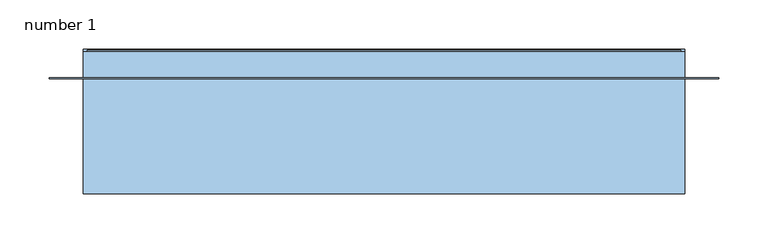
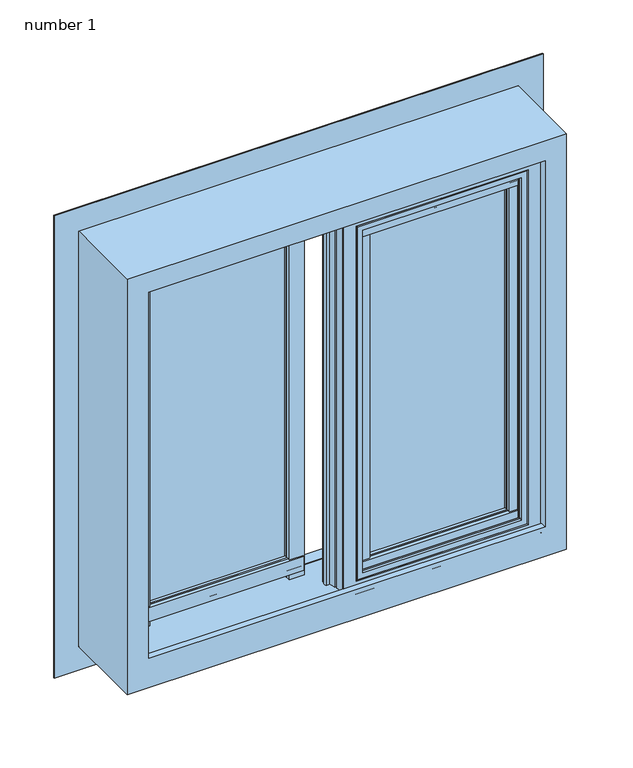
"""IFC4 building model written with IfcOpenShell, lengths in millimetres: window geometry, Window-Exterior-Sierra-Horizontal_Sliding_XO-36inch_Width-Standard : number 1."""

from ifc_helpers import new_model, si_unit, point, frame, frame_2d, origin, place, context, project, spatial, polyline, circle_curve, ellipse_curve, trimmed, segment, composite_curve, outline, extrude, faceted_brep, source, transform, mapped, element, save
from ifc_brep_helpers import plane_surface, cylinder_surface, revolved_surface, advanced_brep


def number_1_ea4afa80(model_context):
    return source(origin(), model_context, "Body", "SolidModel", [
        extrude(outline(polyline([(-30.95625, 959.3990662), (-42.06875, 960.3157287), (-42.06875, 980.7896808), (-30.95625, 981.7063433), (-30.95625, 959.3990662)])), frame((23.8125, 0.0, 0.0), z_axis=(1.0, 0.0, 0.0), x_axis=(0.0, 1.0, 0.0)), (0.0, 0.0, 1.0), 231.775),
        extrude(outline(polyline([(-11.90625, 981.7063433), (-0.6945312, 980.9337774), (-0.6945312, 960.1716321), (-11.90625, 959.3990662), (-11.90625, 981.7063433)])), frame((23.8125, 0.0, 0.0), z_axis=(1.0, 0.0, 0.0), x_axis=(0.0, 1.0, 0.0)), (0.0, 0.0, 1.0), 231.775),
        extrude(outline(composite_curve([segment(polyline([(-30.95625, 970.5465365), (-30.95625, 959.4453125), (-33.62325, 959.4453125), (-33.62325, 961.0201125)]), True, "CONTINUOUS"), segment(trimmed(circle_curve(frame_2d((-31.4860105, 966.253572)), 5.6530426), [point((-33.62325, 961.0201125))], [point((-37.12845, 966.5996458))], False, "CARTESIAN"), True, "CONTINUOUS"), segment(polyline([(-37.12845, 966.5996458), (-41.275, 966.5996458), (-41.275, 974.5159792), (-39.5097, 974.5159792)]), True, "CONTINUOUS"), segment(trimmed(circle_curve(frame_2d((-31.4860105, 974.862053)), 8.0311494), [point((-39.5097, 974.5159792))], [point((-37.5778298, 980.0955125))], False, "CARTESIAN"), True, "CONTINUOUS"), segment(polyline([(-37.5778298, 980.0955125), (-37.5778298, 981.6703125), (-30.95625, 981.6703125), (-30.95625, 970.5465365)]), True, "CONTINUOUS")], self_intersect=False)), frame((23.8125, 0.0, 0.0), z_axis=(1.0, 0.0, 0.0), x_axis=(0.0, 1.0, 0.0)), (0.0, 0.0, 1.0), 231.775),
        extrude(outline(polyline([(13.890625, 959.3990662), (2.778125, 960.3157287), (2.778125, 980.7896808), (13.890625, 981.7063433), (13.890625, 959.3990662)])), frame((-255.5875, 0.0, 0.0), z_axis=(1.0, 0.0, 0.0), x_axis=(0.0, 1.0, 0.0)), (0.0, 0.0, 1.0), 231.775),
        extrude(outline(polyline([(32.940625, 981.7063433), (44.1523438, 980.9337774), (44.1523438, 960.1716321), (32.940625, 959.3990662), (32.940625, 981.7063433)])), frame((-255.5875, 0.0, 0.0), z_axis=(1.0, 0.0, 0.0), x_axis=(0.0, 1.0, 0.0)), (0.0, 0.0, 1.0), 231.775),
        extrude(outline(composite_curve([segment(polyline([(13.890625, 970.5465365), (13.890625, 959.4453125), (11.223625, 959.4453125), (11.223625, 961.0201125)]), True, "CONTINUOUS"), segment(trimmed(circle_curve(frame_2d((13.3608645, 966.253572)), 5.6530426), [point((11.223625, 961.0201125))], [point((7.718425, 966.5996458))], False, "CARTESIAN"), True, "CONTINUOUS"), segment(polyline([(7.718425, 966.5996458), (3.571875, 966.5996458), (3.571875, 974.5159792), (5.337175, 974.5159792)]), True, "CONTINUOUS"), segment(trimmed(circle_curve(frame_2d((13.3608645, 974.862053)), 8.0311494), [point((5.337175, 974.5159792))], [point((7.2690452, 980.0955125))], False, "CARTESIAN"), True, "CONTINUOUS"), segment(polyline([(7.2690452, 980.0955125), (7.2690452, 981.6703125), (13.890625, 981.6703125), (13.890625, 970.5465365)]), True, "CONTINUOUS")], self_intersect=False)), frame((-255.5875, 0.0, 0.0), z_axis=(1.0, 0.0, 0.0), x_axis=(0.0, 1.0, 0.0)), (0.0, 0.0, 1.0), 231.775),
        extrude(outline(polyline([(13.890625, 1456.6834412), (2.778125, 1457.6001037), (2.778125, 1478.0740558), (13.890625, 1478.9907183), (13.890625, 1456.6834412)])), frame((-255.5875, 0.0, 0.0), z_axis=(1.0, 0.0, 0.0), x_axis=(0.0, 1.0, 0.0)), (0.0, 0.0, 1.0), 231.775),
        extrude(outline(polyline([(32.940625, 1478.9907183), (44.1523438, 1478.2181524), (44.1523438, 1457.4560071), (32.940625, 1456.6834412), (32.940625, 1478.9907183)])), frame((-255.5875, 0.0, 0.0), z_axis=(1.0, 0.0, 0.0), x_axis=(0.0, 1.0, 0.0)), (0.0, 0.0, 1.0), 231.775),
        extrude(outline(composite_curve([segment(polyline([(13.890625, 1467.8309115), (13.890625, 1456.7296875), (11.223625, 1456.7296875), (11.223625, 1458.3044875)]), True, "CONTINUOUS"), segment(trimmed(circle_curve(frame_2d((13.3608645, 1463.537947)), 5.6530426), [point((11.223625, 1458.3044875))], [point((7.718425, 1463.8840208))], False, "CARTESIAN"), True, "CONTINUOUS"), segment(polyline([(7.718425, 1463.8840208), (3.571875, 1463.8840208), (3.571875, 1471.8003542), (5.337175, 1471.8003542)]), True, "CONTINUOUS"), segment(trimmed(circle_curve(frame_2d((13.3608645, 1472.146428)), 8.0311494), [point((5.337175, 1471.8003542))], [point((7.2690452, 1477.3798875))], False, "CARTESIAN"), True, "CONTINUOUS"), segment(polyline([(7.2690452, 1477.3798875), (7.2690452, 1478.9546875), (13.890625, 1478.9546875), (13.890625, 1467.8309115)]), True, "CONTINUOUS")], self_intersect=False)), frame((-255.5875, 0.0, 0.0), z_axis=(1.0, 0.0, 0.0), x_axis=(0.0, 1.0, 0.0)), (0.0, 0.0, 1.0), 231.775),
        extrude(outline(polyline([(-30.95625, 1456.6834412), (-42.06875, 1457.6001037), (-42.06875, 1478.0740558), (-30.95625, 1478.9907183), (-30.95625, 1456.6834412)])), frame((23.8125, 0.0, 0.0), z_axis=(1.0, 0.0, 0.0), x_axis=(0.0, 1.0, 0.0)), (0.0, 0.0, 1.0), 231.775),
        extrude(outline(polyline([(-11.90625, 1478.9907183), (-0.6945312, 1478.2181524), (-0.6945312, 1457.4560071), (-11.90625, 1456.6834412), (-11.90625, 1478.9907183)])), frame((23.8125, 0.0, 0.0), z_axis=(1.0, 0.0, 0.0), x_axis=(0.0, 1.0, 0.0)), (0.0, 0.0, 1.0), 231.775),
        extrude(outline(composite_curve([segment(polyline([(-30.95625, 1467.8309115), (-30.95625, 1456.7296875), (-33.62325, 1456.7296875), (-33.62325, 1458.3044875)]), True, "CONTINUOUS"), segment(trimmed(circle_curve(frame_2d((-31.4860105, 1463.537947)), 5.6530426), [point((-33.62325, 1458.3044875))], [point((-37.12845, 1463.8840208))], False, "CARTESIAN"), True, "CONTINUOUS"), segment(polyline([(-37.12845, 1463.8840208), (-41.275, 1463.8840208), (-41.275, 1471.8003542), (-39.5097, 1471.8003542)]), True, "CONTINUOUS"), segment(trimmed(circle_curve(frame_2d((-31.4860105, 1472.146428)), 8.0311494), [point((-39.5097, 1471.8003542))], [point((-37.5778298, 1477.3798875))], False, "CARTESIAN"), True, "CONTINUOUS"), segment(polyline([(-37.5778298, 1477.3798875), (-37.5778298, 1478.9546875), (-30.95625, 1478.9546875), (-30.95625, 1467.8309115)]), True, "CONTINUOUS")], self_intersect=False)), frame((23.8125, 0.0, 0.0), z_axis=(1.0, 0.0, 0.0), x_axis=(0.0, 1.0, 0.0)), (0.0, 0.0, 1.0), 231.775),
        extrude(outline(polyline([(-258.2134338, 13.890625), (-235.9061567, 13.890625), (-236.8228192, 4.365625), (-257.2967713, 4.365625), (-258.2134338, 13.890625)])), frame((0.0, 0.0, 952.5), z_axis=(0.0, 0.0, 1.0), x_axis=(1.0, 0.0, 0.0)), (0.0, 0.0, 1.0), 533.4),
        extrude(outline(polyline([(-235.9061567, 32.940625), (-258.2134338, 32.940625), (-257.4408679, 42.5648438), (-236.6787226, 42.5648438), (-235.9061567, 32.940625)])), frame((0.0, 0.0, 952.5), z_axis=(0.0, 0.0, 1.0), x_axis=(1.0, 0.0, 0.0)), (0.0, 0.0, 1.0), 533.4),
        extrude(outline(composite_curve([segment(polyline([(-247.0659635, 13.890625), (-235.9421875, 13.890625), (-235.9421875, 9.5985242), (-237.5169875, 9.5985242)]), True, "CONTINUOUS"), segment(trimmed(circle_curve(frame_2d((-242.750447, 13.3608645)), 6.445487), [point((-237.5169875, 9.5985242))], [point((-243.0965208, 6.924675))], False, "CARTESIAN"), True, "CONTINUOUS"), segment(polyline([(-243.0965208, 6.924675), (-243.0965208, 5.159375), (-251.0128542, 5.159375), (-251.0128542, 7.718425)]), True, "CONTINUOUS"), segment(trimmed(circle_curve(frame_2d((-251.358928, 13.3608645)), 5.6530426), [point((-251.0128542, 7.718425))], [point((-256.5923875, 11.223625))], False, "CARTESIAN"), True, "CONTINUOUS"), segment(polyline([(-256.5923875, 11.223625), (-258.1671875, 11.223625), (-258.1671875, 13.890625), (-247.0659635, 13.890625)]), True, "CONTINUOUS")], self_intersect=False)), frame((0.0, 0.0, 952.5), z_axis=(0.0, 0.0, 1.0), x_axis=(1.0, 0.0, 0.0)), (0.0, 0.0, 1.0), 533.4),
        extrude(outline(polyline([(258.2134338, -30.95625), (257.2967713, -40.48125), (236.8228192, -40.48125), (235.9061567, -30.95625), (258.2134338, -30.95625)])), frame((0.0, 0.0, 952.5), z_axis=(0.0, 0.0, 1.0), x_axis=(1.0, 0.0, 0.0)), (0.0, 0.0, 1.0), 533.4),
        extrude(outline(polyline([(235.9061567, -11.90625), (236.6787226, -2.2820312), (257.4408679, -2.2820312), (258.2134338, -11.90625), (235.9061567, -11.90625)])), frame((0.0, 0.0, 952.5), z_axis=(0.0, 0.0, 1.0), x_axis=(1.0, 0.0, 0.0)), (0.0, 0.0, 1.0), 533.4),
        extrude(outline(composite_curve([segment(polyline([(247.0659635, -30.95625), (258.1671875, -30.95625), (258.1671875, -33.62325), (256.5923875, -33.62325)]), True, "CONTINUOUS"), segment(trimmed(circle_curve(frame_2d((251.358928, -31.4860105)), 5.6530426), [point((256.5923875, -33.62325))], [point((251.0128542, -37.12845))], False, "CARTESIAN"), True, "CONTINUOUS"), segment(polyline([(251.0128542, -37.12845), (251.0128542, -39.6875), (243.0965208, -39.6875), (243.0965208, -37.9222)]), True, "CONTINUOUS"), segment(trimmed(circle_curve(frame_2d((242.750447, -31.4860105)), 6.445487), [point((243.0965208, -37.9222))], [point((237.5169875, -35.2483508))], False, "CARTESIAN"), True, "CONTINUOUS"), segment(polyline([(237.5169875, -35.2483508), (235.9421875, -35.2483508), (235.9421875, -30.95625), (247.0659635, -30.95625)]), True, "CONTINUOUS")], self_intersect=False)), frame((0.0, 0.0, 952.5), z_axis=(0.0, 0.0, 1.0), x_axis=(1.0, 0.0, 0.0)), (0.0, 0.0, 1.0), 533.4),
        extrude(outline(polyline([(879.8514818, 339.3495838), (1558.5495838, 339.3495838), (1558.5495838, -339.3495838), (879.8514818, -339.3495838), (879.8514818, 339.3495838)]), holes=[polyline([(914.4200683, -304.7809972), (1523.9809972, -304.7809972), (1523.9809972, 304.7809972), (914.4200683, 304.7809972), (914.4200683, -304.7809972)])]), frame((0.0, 56.35625, 0.0), z_axis=(0.0, 1.0, 0.0), x_axis=(0.0, 0.0, 1.0)), (0.0, 0.0, 1.0), 1.3692925),
        faceted_brep([(287.4452673, 61.8007595, 1506.6452673), (289.7632068, 85.439324, 1508.9632068), (289.7632068, 85.439324, 915.510409), (287.4452673, 61.8007595, 915.510409), (-287.4452673, 61.8007595, 1506.6452673), (-289.7632068, 85.439324, 1508.9632068), (-304.8, -59.8487004, 1524.0), (304.8, -59.8487004, 1524.0), (304.8, 83.8857584, 1524.0), (-304.8, 83.8857584, 1524.0), (-287.4452673, 61.8007595, 915.510409), (-289.7632068, 85.439324, 915.510409), (275.3297286, -59.8487004, 1494.5297286), (275.3297286, -48.9537259, 1494.5297286), (275.3297286, -48.9537259, 950.6555073), (275.3297286, -50.9012589, 951.1326574), (275.3297286, -50.9012589, 957.3267373), (275.3297286, -59.8487004, 957.3267373), (287.8836, -48.9537259, 1507.0836), (287.8836, -1.4525069, 1507.0836), (287.8836, -1.4525069, 939.0175967), (287.8836, -48.9537259, 950.6555073), (278.7400777, -1.4525069, 1497.9400777), (278.7400777, 10.1171482, 1497.9400777), (278.7400777, 10.1171482, 936.1830039), (278.7400777, -1.4525069, 939.0175967), (273.6551976, 10.1171482, 1492.8551976), (273.6551976, 26.899095, 1492.8551976), (273.6551976, 26.899095, 932.0713873), (273.6551976, 10.1171482, 936.1830039), (-304.8, 83.8857584, 915.510409), (-304.8, 86.3576576, 915.510409), (-304.8, 86.3576576, 914.4), (-304.8, -59.8487004, 914.4), (304.8, -59.8487004, 914.4), (304.8, 86.3576576, 914.4), (304.8, 86.3576576, 915.510409), (304.8, 83.8857584, 915.510409), (-275.3297286, -59.8487004, 1494.5297286), (-275.3297286, -59.8487004, 957.3267373), (-275.3297286, -50.9012589, 957.3267373), (-275.3297286, -50.9012589, 951.1326574), (278.8170827, 26.899095, 932.0713873), (278.8170827, 39.894466, 928.8874908), (269.0057011, 41.2733658, 928.5496571), (268.4593437, 52.0255869, 925.9153376), (277.5829219, 52.0255869, 925.9153376), (277.5829219, 55.096925, 925.1628525), (273.177436, 55.096925, 925.1628525), (273.177436, 56.33085, 924.860538), (-273.177436, 56.3169605, 924.8639409), (-273.177436, 55.096925, 925.1628525), (-277.5829219, 55.096925, 925.1628525), (-277.5829219, 52.0255869, 925.9153376), (-268.4593437, 52.0255869, 925.9153376), (-269.0057011, 41.2733658, 928.5496571), (-278.8170827, 39.894466, 928.8874908), (-278.8170827, 26.899095, 932.0713873), (-273.6551976, 26.899095, 932.0713873), (-273.6551976, 10.1171482, 936.1830039), (-278.7400777, 10.1171482, 936.1830039), (-278.7400777, -1.4525069, 939.0175967), (-287.8836, -1.4525069, 939.0175967), (-287.8836, -48.9537259, 950.6555073), (-275.3297286, -48.9537259, 950.6555073), (273.177436, 57.6604904, 924.8639409), (-273.177436, 57.6604904, 924.8639409), (273.177436, 57.6604904, 915.510409), (-273.177436, 57.6604904, 915.510409), (-275.3297286, -48.9537259, 1494.5297286), (-287.8836, -48.9537259, 1507.0836), (-287.8836, -1.4525069, 1507.0836), (-278.7400777, -1.4525069, 1497.9400777), (-278.7400777, 10.1171482, 1497.9400777), (-273.6551976, 10.1171482, 1492.8551976), (-273.6551976, 26.899095, 1492.8551976), (-278.8170827, 26.899095, 1498.0170827), (278.8170827, 26.899095, 1498.0170827), (278.8170827, 39.894466, 1498.0170827), (269.0057011, 41.2733658, 1488.2057011), (-278.8170827, 39.894466, 1498.0170827), (-301.117, 85.439324, 915.510409), (-301.117, 85.439324, 1520.317), (301.117, 85.439324, 1520.317), (301.117, 85.439324, 915.510409), (301.117, 77.5357584, 1520.317), (301.117, 77.5357584, 915.510409), (-301.117, 77.5357584, 1520.317), (-301.117, 77.5357584, 915.510409), (-303.403, 77.5357584, 915.510409), (-303.403, 77.5357584, 1522.603), (303.403, 77.5357584, 1522.603), (303.403, 77.5357584, 915.510409), (303.403, 83.8857584, 1522.603), (303.403, 83.8857584, 915.510409), (-303.403, 83.8857584, 1522.603), (-303.403, 83.8857584, 915.510409), (-279.4071742, 61.8007595, 915.510409), (-279.4071742, 60.6800805, 915.510409), (-273.177436, 60.6800805, 915.510409), (273.177436, 60.6800805, 915.510409), (279.4071742, 60.6800805, 915.510409), (279.4071742, 61.8007595, 915.510409), (-269.0057011, 41.2733658, 1488.2057011), (268.4593437, 52.0255869, 1487.6593437), (-268.4593437, 52.0255869, 1487.6593437), (-277.5829219, 52.0255869, 1496.7829219), (277.5829219, 52.0255869, 1496.7829219), (277.5829219, 55.096925, 1496.7829219), (-277.5829219, 55.096925, 1496.7829219), (-273.177436, 55.096925, 1492.377436), (273.177436, 55.096925, 1492.377436), (273.177436, 60.6800805, 1492.377436), (-273.177436, 60.6800805, 1492.377436), (-279.4071742, 60.6800805, 1498.6071742), (279.4071742, 60.6800805, 1498.6071742), (279.4071742, 61.8007595, 1498.6071742), (-279.4071742, 61.8007595, 1498.6071742)], [[[0, 1, 2, 3]], [[1, 0, 4, 5]], [[6, 7, 8, 9]], [[5, 4, 10, 11]], [[12, 13, 14, 15, 16, 17]], [[18, 19, 20, 21]], [[22, 23, 24, 25]], [[26, 27, 28, 29]], [[6, 9, 30, 31, 32, 33]], [[8, 7, 34, 35, 36, 37]], [[35, 34, 33, 32]], [[7, 6, 33, 34], [38, 12, 17, 39]], [[39, 17, 16, 40]], [[40, 16, 15, 41]], [[41, 15, 14, 21, 20, 25, 24, 29, 28, 42, 43, 44, 45, 46, 47, 48, 49, 50, 51, 52, 53, 54, 55, 56, 57, 58, 59, 60, 61, 62, 63, 64]], [[65, 66, 50, 49]], [[66, 65, 67, 68]], [[13, 69, 64, 63, 70, 18, 21, 14]], [[19, 71, 62, 61, 72, 22, 25, 20]], [[23, 73, 60, 59, 74, 26, 29, 24]], [[27, 75, 58, 57, 76, 77, 42, 28]], [[77, 78, 43, 42]], [[78, 79, 44, 43]], [[12, 38, 69, 13]], [[18, 70, 71, 19]], [[22, 72, 73, 23]], [[26, 74, 75, 27]], [[77, 76, 80, 78]], [[69, 38, 39, 40, 41, 64]], [[71, 70, 63, 62]], [[73, 72, 61, 60]], [[75, 74, 59, 58]], [[80, 76, 57, 56]], [[1, 5, 11, 81, 82, 83, 84, 2]], [[83, 85, 86, 84]], [[85, 87, 88, 89, 90, 91, 92, 86]], [[91, 93, 94, 92]], [[9, 8, 37, 94, 93, 95, 96, 30]], [[83, 82, 87, 85]], [[91, 90, 95, 93]], [[87, 82, 81, 88]], [[95, 90, 89, 96]], [[36, 31, 30, 96, 89, 88, 81, 11, 10, 97, 98, 99, 68, 67, 100, 101, 102, 3, 2, 84, 86, 92, 94, 37]], [[32, 31, 36, 35]], [[79, 78, 80, 103]], [[103, 80, 56, 55]], [[79, 104, 45, 44]], [[104, 105, 54, 53, 106, 107, 46, 45]], [[107, 108, 47, 46]], [[108, 109, 52, 51, 110, 111, 48, 47]], [[111, 112, 100, 67, 65, 49, 48]], [[112, 113, 99, 98, 114, 115, 101, 100]], [[115, 116, 102, 101]], [[4, 0, 3, 102, 116, 117, 97, 10]], [[79, 103, 105, 104]], [[107, 106, 109, 108]], [[111, 110, 113, 112]], [[115, 114, 117, 116]], [[105, 103, 55, 54]], [[109, 106, 53, 52]], [[113, 110, 51, 50, 66, 68, 99]], [[117, 114, 98, 97]]]),
        extrude(outline(polyline([(43.5040588, -30.95625), (42.5873963, -40.48125), (22.1134442, -40.48125), (21.1967817, -30.95625), (43.5040588, -30.95625)])), frame((0.0, 0.0, 952.5), z_axis=(0.0, 0.0, 1.0), x_axis=(1.0, 0.0, 0.0)), (0.0, 0.0, 1.0), 533.4),
        extrude(outline(polyline([(21.1967817, -11.90625), (21.9693476, -2.2820312), (42.7314929, -2.2820312), (43.5040588, -11.90625), (21.1967817, -11.90625)])), frame((0.0, 0.0, 952.5), z_axis=(0.0, 0.0, 1.0), x_axis=(1.0, 0.0, 0.0)), (0.0, 0.0, 1.0), 533.4),
        extrude(outline(composite_curve([segment(polyline([(32.3565885, -30.95625), (43.4578125, -30.95625), (43.4578125, -33.62325), (41.8830125, -33.62325)]), True, "CONTINUOUS"), segment(trimmed(circle_curve(frame_2d((36.649553, -31.4860105)), 5.6530426), [point((41.8830125, -33.62325))], [point((36.3034792, -37.12845))], False, "CARTESIAN"), True, "CONTINUOUS"), segment(polyline([(36.3034792, -37.12845), (36.3034792, -39.6875), (28.3871458, -39.6875), (28.3871458, -37.9222)]), True, "CONTINUOUS"), segment(trimmed(circle_curve(frame_2d((28.041072, -31.4860105)), 6.445487), [point((28.3871458, -37.9222))], [point((22.8076125, -35.2483508))], False, "CARTESIAN"), True, "CONTINUOUS"), segment(polyline([(22.8076125, -35.2483508), (21.2328125, -35.2483508), (21.2328125, -30.95625), (32.3565885, -30.95625)]), True, "CONTINUOUS")], self_intersect=False)), frame((0.0, 0.0, 952.5), z_axis=(0.0, 0.0, 1.0), x_axis=(1.0, 0.0, 0.0)), (0.0, 0.0, 1.0), 533.4),
        extrude(outline(polyline([(-43.5040588, 13.890625), (-21.1967817, 13.890625), (-22.1134442, 4.365625), (-42.5873963, 4.365625), (-43.5040588, 13.890625)])), frame((0.0, 0.0, 952.5), z_axis=(0.0, 0.0, 1.0), x_axis=(1.0, 0.0, 0.0)), (0.0, 0.0, 1.0), 533.4),
        extrude(outline(polyline([(-21.1967817, 32.940625), (-43.5040588, 32.940625), (-42.7314929, 42.5648438), (-21.9693476, 42.5648438), (-21.1967817, 32.940625)])), frame((0.0, 0.0, 952.5), z_axis=(0.0, 0.0, 1.0), x_axis=(1.0, 0.0, 0.0)), (0.0, 0.0, 1.0), 533.4),
        extrude(outline(composite_curve([segment(polyline([(-32.3565885, 13.890625), (-21.2328125, 13.890625), (-21.2328125, 9.5985242), (-22.8076125, 9.5985242)]), True, "CONTINUOUS"), segment(trimmed(circle_curve(frame_2d((-28.041072, 13.3608645)), 6.445487), [point((-22.8076125, 9.5985242))], [point((-28.3871458, 6.924675))], False, "CARTESIAN"), True, "CONTINUOUS"), segment(polyline([(-28.3871458, 6.924675), (-28.3871458, 5.159375), (-36.3034792, 5.159375), (-36.3034792, 7.718425)]), True, "CONTINUOUS"), segment(trimmed(circle_curve(frame_2d((-36.649553, 13.3608645)), 5.6530426), [point((-36.3034792, 7.718425))], [point((-41.8830125, 11.223625))], False, "CARTESIAN"), True, "CONTINUOUS"), segment(polyline([(-41.8830125, 11.223625), (-43.4578125, 11.223625), (-43.4578125, 13.890625), (-32.3565885, 13.890625)]), True, "CONTINUOUS")], self_intersect=False)), frame((0.0, 0.0, 952.5), z_axis=(0.0, 0.0, 1.0), x_axis=(1.0, 0.0, 0.0)), (0.0, 0.0, 1.0), 533.4),
        extrude(outline(polyline([(258.95935, -11.90625), (258.95935, -30.955332), (20.44065, -30.955332), (20.44065, -11.90625), (258.95935, -11.90625)])), frame((0.0, 0.0, 958.65315), z_axis=(0.0, 0.0, 1.0), x_axis=(1.0, 0.0, 0.0)), (0.0, 0.0, 1.0), 521.0937),
        advanced_brep(
        [(250.12015, -9.74725, 967.49235), (29.27985, -9.74725, 967.49235), (29.27985, -10.8831079, 967.49235), (250.12015, -10.8831079, 967.49235), (248.2833265, -7.3042106, 969.3291735), (31.1166735, -7.3042106, 969.3291735), (31.3062238, -9.74725, 969.5187238), (248.0937762, -9.74725, 969.5187238), (256.08915, -4.76885, 961.52335), (23.31085, -4.76885, 961.52335), (256.08915, -2.38125, 961.52335), (23.31085, -2.38125, 961.52335), (280.77795, -4.76885, 936.83455), (-1.37795, -4.76885, 936.83455), (1.00965, -2.38125, 939.22215), (278.39035, -2.38125, 939.22215), (280.77795, -7.33425, 936.83455), (-1.37795, -7.33425, 936.83455), (278.74595, -9.01065, 938.86655), (0.65405, -9.01065, 938.86655), (0.65405, -7.33425, 938.86655), (278.74595, -7.33425, 938.86655), (275.44395, -10.91565, 942.16855), (3.95605, -10.91565, 942.16855), (3.95605, -9.01065, 942.16855), (275.44395, -9.01065, 942.16855), (283.36875, -16.52905, 934.24375), (-3.96875, -16.52905, 934.24375), (-3.96875, -10.91565, 934.24375), (283.36875, -10.91565, 934.24375), (278.06015, -28.72105, 939.55235), (1.33985, -28.72105, 939.55235), (1.33985, -16.52905, 939.55235), (278.06015, -16.52905, 939.55235), (278.06015, -32.68345, 939.55235), (1.33985, -32.68345, 939.55235), (278.06015, -46.01845, 939.55235), (1.33985, -46.01845, 939.55235), (277.24735, -46.83125, 940.36515), (2.15265, -46.83125, 940.36515), (258.95935, -44.950732, 958.65315), (20.44065, -44.950732, 958.65315), (20.44065, -46.83125, 958.65315), (258.95935, -46.83125, 958.65315), (257.3584612, -46.550932, 960.2540388), (22.0415388, -46.550932, 960.2540388), (22.0415388, -44.950732, 960.2540388), (257.3584612, -44.950732, 960.2540388), (249.8146612, -42.7830125, 967.7978388), (29.5853388, -42.7830125, 967.7978388), (29.5853388, -46.550932, 967.7978388), (249.8146612, -46.550932, 967.7978388), (246.6396612, -30.955332, 970.9728388), (32.7603388, -30.955332, 970.9728388), (31.7476888, -42.7830125, 969.9601888), (247.6523112, -42.7830125, 969.9601888), (258.95935, -33.3436209, 958.65315), (20.44065, -33.3436209, 958.65315), (22.8289388, -30.955332, 961.0414388), (256.5710612, -30.955332, 961.0414388), (258.95935, -11.90625, 958.65315), (20.44065, -11.90625, 958.65315), (254.3555891, -10.8831079, 963.2569109), (25.0444109, -10.8831079, 963.2569109), (24.0212688, -11.90625, 962.2337688), (255.3787312, -11.90625, 962.2337688), (29.27985, -9.74725, 1470.90765), (29.27985, -10.8831079, 1470.90765), (31.1166735, -7.3042106, 1469.0708265), (31.3062238, -9.74725, 1468.8812762), (23.31085, -4.76885, 1476.87665), (23.31085, -2.38125, 1476.87665), (-1.37795, -4.76885, 1501.56545), (1.00965, -2.38125, 1499.17785), (-1.37795, -7.33425, 1501.56545), (0.65405, -9.01065, 1499.53345), (0.65405, -7.33425, 1499.53345), (3.95605, -10.91565, 1496.23145), (3.95605, -9.01065, 1496.23145), (-3.96875, -16.52905, 1504.15625), (-3.96875, -10.91565, 1504.15625), (1.33985, -28.72105, 1498.84765), (1.33985, -16.52905, 1498.84765), (1.33985, -32.68345, 1498.84765), (1.33985, -46.01845, 1498.84765), (2.15265, -46.83125, 1498.03485), (20.44065, -44.950732, 1479.74685), (20.44065, -46.83125, 1479.74685), (22.0415388, -46.550932, 1478.1459612), (22.0415388, -44.950732, 1478.1459612), (29.5853388, -42.7830125, 1470.6021612), (29.5853388, -46.550932, 1470.6021612), (32.7603388, -30.955332, 1467.4271612), (31.7476888, -42.7830125, 1468.4398112), (20.44065, -33.3436209, 1479.74685), (22.8289388, -30.955332, 1477.3585612), (20.44065, -11.90625, 1479.74685), (25.0444109, -10.8831079, 1475.1430891), (24.0212688, -11.90625, 1476.1662312), (250.12015, -9.74725, 1470.90765), (250.12015, -10.8831079, 1470.90765), (248.2833265, -7.3042106, 1469.0708265), (248.0937762, -9.74725, 1468.8812762), (256.08915, -4.76885, 1476.87665), (256.08915, -2.38125, 1476.87665), (280.77795, -4.76885, 1501.56545), (278.39035, -2.38125, 1499.17785), (280.77795, -7.33425, 1501.56545), (278.74595, -9.01065, 1499.53345), (278.74595, -7.33425, 1499.53345), (275.44395, -10.91565, 1496.23145), (275.44395, -9.01065, 1496.23145), (283.36875, -16.52905, 1504.15625), (283.36875, -10.91565, 1504.15625), (278.06015, -28.72105, 1498.84765), (278.06015, -16.52905, 1498.84765), (278.06015, -32.68345, 1498.84765), (278.06015, -46.01845, 1498.84765), (277.24735, -46.83125, 1498.03485), (258.95935, -44.950732, 1479.74685), (258.95935, -46.83125, 1479.74685), (257.3584612, -46.550932, 1478.1459612), (257.3584612, -44.950732, 1478.1459612), (249.8146612, -42.7830125, 1470.6021612), (249.8146612, -46.550932, 1470.6021612), (246.6396612, -30.955332, 1467.4271612), (247.6523112, -42.7830125, 1468.4398112), (258.95935, -33.3436209, 1479.74685), (256.5710612, -30.955332, 1477.3585612), (258.95935, -11.90625, 1479.74685), (254.3555891, -10.8831079, 1475.1430891), (255.3787312, -11.90625, 1476.1662312)],
        [
            (0, 1),
            (1, 2),
            (2, 3),
            (3, 0),
            (4, 5),
            (5, 6),
            (6, 7),
            (7, 4),
            (8, 9),
            (9, 5),
            (4, 8),
            (10, 11),
            (11, 9),
            (8, 10),
            (12, 13),
            (13, 14, ellipse_curve(frame((1.00965, -4.76885, 939.22215), z_axis=(0.7071067811865475, 0.0, -0.7071067811865475), x_axis=(0.7071067811865476, 0.0, 0.7071067811865474)), 3.3765763, 2.3876)),
            (14, 15),
            (15, 12, ellipse_curve(frame((278.39035, -4.76885, 939.22215), z_axis=(-0.7071067811865475, 0.0, -0.7071067811865475), x_axis=(0.7071067811865476, 0.0, -0.7071067811865474)), 3.3765763, 2.3876)),
            (16, 17),
            (17, 13),
            (12, 16),
            (18, 19),
            (19, 20),
            (20, 21),
            (21, 18),
            (22, 23),
            (23, 24),
            (24, 25),
            (25, 22),
            (26, 27),
            (27, 28),
            (28, 29),
            (29, 26),
            (30, 31),
            (31, 32),
            (32, 33),
            (33, 30),
            (34, 35),
            (35, 31, ellipse_curve(frame((1.33985, -30.70225, 939.55235), z_axis=(-0.7071067811865475, 0.0, 0.7071067811865475), x_axis=(-0.7071067811865476, 0.0, -0.7071067811865474)), 2.8018399, 1.9812)),
            (30, 34, ellipse_curve(frame((278.06015, -30.70225, 939.55235), z_axis=(0.7071067811865475, 0.0, 0.7071067811865475), x_axis=(-0.7071067811865476, 0.0, 0.7071067811865474)), 2.8018399, 1.9812)),
            (36, 37),
            (37, 35),
            (34, 36),
            (38, 39),
            (39, 37, ellipse_curve(frame((2.15265, -46.01845, 940.36515), z_axis=(0.7071067811865475, 0.0, -0.7071067811865475), x_axis=(0.7071067811865476, 0.0, 0.7071067811865474)), 1.1494728, 0.8128)),
            (36, 38, ellipse_curve(frame((277.24735, -46.01845, 940.36515), z_axis=(-0.7071067811865475, 0.0, -0.7071067811865475), x_axis=(0.7071067811865476, 0.0, -0.7071067811865474)), 1.1494728, 0.8128)),
            (40, 41),
            (41, 42),
            (42, 43),
            (43, 40),
            (44, 45),
            (45, 46),
            (46, 47),
            (47, 44),
            (48, 49),
            (49, 50),
            (50, 51),
            (51, 48),
            (52, 53),
            (53, 54),
            (54, 55),
            (55, 52),
            (56, 57),
            (57, 58),
            (58, 59),
            (59, 56),
            (60, 61),
            (61, 57),
            (56, 60),
            (62, 63),
            (63, 64),
            (64, 65),
            (65, 62),
            (1, 66),
            (66, 67),
            (67, 2),
            (5, 68),
            (68, 69),
            (69, 6),
            (9, 70),
            (70, 68),
            (11, 71),
            (71, 70),
            (13, 72),
            (72, 73, ellipse_curve(frame((1.00965, -4.76885, 1499.17785), z_axis=(-0.7071067811865475, 0.0, -0.7071067811865475), x_axis=(0.7071067811865474, 0.0, -0.7071067811865476)), 3.3765763, 2.3876)),
            (73, 14),
            (17, 74),
            (74, 72),
            (19, 75),
            (75, 76),
            (76, 20),
            (23, 77),
            (77, 78),
            (78, 24),
            (27, 79),
            (79, 80),
            (80, 28),
            (31, 81),
            (81, 82),
            (82, 32),
            (35, 83),
            (83, 81, ellipse_curve(frame((1.33985, -30.70225, 1498.84765), z_axis=(0.7071067811865475, 0.0, 0.7071067811865475), x_axis=(-0.7071067811865474, 0.0, 0.7071067811865476)), 2.8018399, 1.9812)),
            (37, 84),
            (84, 83),
            (39, 85),
            (85, 84, ellipse_curve(frame((2.15265, -46.01845, 1498.03485), z_axis=(-0.7071067811865475, 0.0, -0.7071067811865475), x_axis=(0.7071067811865474, 0.0, -0.7071067811865476)), 1.1494728, 0.8128)),
            (41, 86),
            (86, 87),
            (87, 42),
            (45, 88),
            (88, 89),
            (89, 46),
            (49, 90),
            (90, 91),
            (91, 50),
            (53, 92),
            (92, 93),
            (93, 54),
            (57, 94),
            (94, 95),
            (95, 58),
            (61, 96),
            (96, 94),
            (63, 97),
            (97, 98),
            (98, 64),
            (66, 99),
            (99, 100),
            (100, 67),
            (68, 101),
            (101, 102),
            (102, 69),
            (70, 103),
            (103, 101),
            (71, 104),
            (104, 103),
            (72, 105),
            (105, 106, ellipse_curve(frame((278.39035, -4.76885, 1499.17785), z_axis=(-0.7071067811865475, 0.0, 0.7071067811865475), x_axis=(-0.7071067811865476, 0.0, -0.7071067811865474)), 3.3765763, 2.3876)),
            (106, 73),
            (74, 107),
            (107, 105),
            (75, 108),
            (108, 109),
            (109, 76),
            (77, 110),
            (110, 111),
            (111, 78),
            (79, 112),
            (112, 113),
            (113, 80),
            (81, 114),
            (114, 115),
            (115, 82),
            (83, 116),
            (116, 114, ellipse_curve(frame((278.06015, -30.70225, 1498.84765), z_axis=(0.7071067811865475, 0.0, -0.7071067811865475), x_axis=(0.7071067811865476, 0.0, 0.7071067811865474)), 2.8018399, 1.9812)),
            (84, 117),
            (117, 116),
            (85, 118),
            (118, 117, ellipse_curve(frame((277.24735, -46.01845, 1498.03485), z_axis=(-0.7071067811865475, 0.0, 0.7071067811865475), x_axis=(-0.7071067811865476, 0.0, -0.7071067811865474)), 1.1494728, 0.8128)),
            (86, 119),
            (119, 120),
            (120, 87),
            (88, 121),
            (121, 122),
            (122, 89),
            (90, 123),
            (123, 124),
            (124, 91),
            (92, 125),
            (125, 126),
            (126, 93),
            (94, 127),
            (127, 128),
            (128, 95),
            (96, 129),
            (129, 127),
            (97, 130),
            (130, 131),
            (131, 98),
            (62, 130),
            (100, 3),
            (99, 0),
            (102, 7),
            (101, 4),
            (103, 8),
            (104, 10),
            (106, 15),
            (105, 12),
            (107, 16),
            (109, 21),
            (108, 18),
            (111, 25),
            (110, 22),
            (113, 29),
            (112, 26),
            (115, 33),
            (114, 30),
            (116, 34),
            (117, 36),
            (118, 38),
            (120, 43),
            (119, 40),
            (122, 47),
            (121, 44),
            (124, 51),
            (123, 48),
            (126, 55),
            (125, 52),
            (128, 59),
            (127, 56),
            (129, 60),
            (131, 65),
        ],
        [
            plane_surface(frame((250.12015, -10.8831079, 967.49235), z_axis=(0.0, 0.0, 1.0), x_axis=(-1.0, 0.0, 0.0))),
            plane_surface(frame((248.0937762, -9.74725, 969.5187238), z_axis=(0.0, 0.07735544009934271, 0.9970035786731345), x_axis=(-1.0, 0.0, 0.0))),
            plane_surface(frame((248.2833265, -7.3042106, 969.3291735), z_axis=(0.0, 0.9510889261909004, 0.3089172291683326), x_axis=(-1.0, 0.0, 0.0))),
            plane_surface(frame((256.08915, -4.76885, 961.52335), z_axis=(0.0, 0.0, 1.0), x_axis=(-1.0, 0.0, 0.0))),
            cylinder_surface(frame((283.36875, -4.76885, 939.22215), z_axis=(1.0, 0.0, 0.0), x_axis=(0.0, -1.0, 0.0)), 2.3876),
            plane_surface(frame((280.77795, -4.76885, 936.83455), z_axis=(0.0, 0.0, -1.0), x_axis=(-1.0, 0.0, 0.0))),
            plane_surface(frame((278.74595, -7.33425, 938.86655), z_axis=(0.0, 0.0, -1.0), x_axis=(-1.0, 0.0, 0.0))),
            plane_surface(frame((275.44395, -9.01065, 942.16855), z_axis=(0.0, 0.0, -1.0), x_axis=(-1.0, 0.0, 0.0))),
            plane_surface(frame((283.36875, -10.91565, 934.24375), z_axis=(0.0, 0.0, -1.0), x_axis=(-1.0, 0.0, 0.0))),
            plane_surface(frame((278.06015, -16.52905, 939.55235), z_axis=(0.0, 0.0, -1.0), x_axis=(-1.0, 0.0, 0.0))),
            revolved_surface(polyline([(-0.6413499930890225, -32.68345, 939.55235), (280.04134999308906, -32.68345, 939.55235)]), (283.36875, -30.70225, 939.55235), (-1.0, 0.0, 0.0)),
            plane_surface(frame((278.06015, -32.68345, 939.55235), z_axis=(0.0, 0.0, -1.0), x_axis=(-1.0, 0.0, 0.0))),
            cylinder_surface(frame((283.36875, -46.01845, 940.36515), z_axis=(1.0, 0.0, 0.0), x_axis=(0.0, -1.0, 0.0)), 0.8128),
            plane_surface(frame((258.95935, -46.83125, 958.65315), z_axis=(0.0, 0.0, 1.0), x_axis=(-1.0, 0.0, 0.0))),
            plane_surface(frame((257.3584612, -44.950732, 960.2540388), z_axis=(0.0, 0.0, -1.0), x_axis=(-1.0, 0.0, 0.0))),
            plane_surface(frame((249.8146612, -46.550932, 967.7978388), z_axis=(0.0, 0.0, 1.0), x_axis=(-1.0, 0.0, 0.0))),
            plane_surface(frame((247.6523112, -42.7830125, 969.9601888), z_axis=(0.0, -0.08530487454184647, 0.996354895797376), x_axis=(-1.0, 0.0, 0.0))),
            plane_surface(frame((256.5710612, -30.955332, 961.0414388), z_axis=(0.0, 0.7071067811865713, -0.7071067811865238), x_axis=(-1.0, 0.0, 0.0))),
            plane_surface(frame((258.95935, -33.3436209, 958.65315), z_axis=(0.0, 0.0, 1.0), x_axis=(-1.0, 0.0, 0.0))),
            plane_surface(frame((255.3787312, -11.90625, 962.2337688), z_axis=(0.0, -0.7071067811861558, 0.7071067811869393), x_axis=(-1.0, 0.0, 0.0))),
            plane_surface(frame((29.27985, -10.8831079, 967.49235), z_axis=(1.0, 0.0, 0.0), x_axis=(0.0, 0.0, 1.0))),
            plane_surface(frame((31.3062238, -9.74725, 969.5187238), z_axis=(0.9970035786731345, 0.07735544009934266, 0.0), x_axis=(0.0, 0.0, 1.0))),
            plane_surface(frame((31.1166735, -7.3042106, 969.3291735), z_axis=(0.30891722916833264, 0.9510889261909004, 0.0), x_axis=(0.0, 0.0, 1.0))),
            plane_surface(frame((23.31085, -4.76885, 961.52335), z_axis=(1.0, 0.0, 0.0), x_axis=(0.0, 0.0, 1.0))),
            cylinder_surface(frame((1.00965, -4.76885, 934.24375), z_axis=(0.0, 0.0, -1.0), x_axis=(0.0, -1.0, 0.0)), 2.3876),
            plane_surface(frame((-1.37795, -4.76885, 936.83455), z_axis=(-1.0, 0.0, 0.0), x_axis=(0.0, 0.0, 1.0))),
            plane_surface(frame((0.65405, -7.33425, 938.86655), z_axis=(-1.0, 0.0, 0.0), x_axis=(0.0, 0.0, 1.0))),
            plane_surface(frame((3.95605, -9.01065, 942.16855), z_axis=(-1.0, 0.0, 0.0), x_axis=(0.0, 0.0, 1.0))),
            plane_surface(frame((-3.96875, -10.91565, 934.24375), z_axis=(-1.0, 0.0, 0.0), x_axis=(0.0, 0.0, 1.0))),
            plane_surface(frame((1.33985, -16.52905, 939.55235), z_axis=(-1.0, 0.0, 0.0), x_axis=(0.0, 0.0, 1.0))),
            revolved_surface(polyline([(1.33985, -32.68345, 1500.828849993089), (1.33985, -32.68345, 937.571150006911)]), (1.33985, -30.70225, 934.24375), (0.0, 0.0, 1.0)),
            plane_surface(frame((1.33985, -32.68345, 939.55235), z_axis=(-1.0, 0.0, 0.0), x_axis=(0.0, 0.0, 1.0))),
            cylinder_surface(frame((2.15265, -46.01845, 934.24375), z_axis=(0.0, 0.0, -1.0), x_axis=(0.0, -1.0, 0.0)), 0.8128),
            plane_surface(frame((20.44065, -46.83125, 958.65315), z_axis=(1.0, 0.0, 0.0), x_axis=(0.0, 0.0, 1.0))),
            plane_surface(frame((22.0415388, -44.950732, 960.2540388), z_axis=(-1.0, 0.0, 0.0), x_axis=(0.0, 0.0, 1.0))),
            plane_surface(frame((29.5853388, -46.550932, 967.7978388), z_axis=(1.0, 0.0, 0.0), x_axis=(0.0, 0.0, 1.0))),
            plane_surface(frame((31.7476888, -42.7830125, 969.9601888), z_axis=(0.996354895797376, -0.08530487454184653, 0.0), x_axis=(0.0, 0.0, 1.0))),
            plane_surface(frame((22.8289388, -30.955332, 961.0414388), z_axis=(-0.7071067811865238, 0.7071067811865713, 0.0), x_axis=(0.0, 0.0, 1.0))),
            plane_surface(frame((20.44065, -33.3436209, 958.65315), z_axis=(1.0, 0.0, 0.0), x_axis=(0.0, 0.0, 1.0))),
            plane_surface(frame((24.0212688, -11.90625, 962.2337688), z_axis=(0.7071067811869393, -0.7071067811861558, 0.0), x_axis=(0.0, 0.0, 1.0))),
            plane_surface(frame((29.27985, -10.8831079, 1470.90765), z_axis=(0.0, 0.0, -1.0), x_axis=(1.0, 0.0, 0.0))),
            plane_surface(frame((31.3062238, -9.74725, 1468.8812762), z_axis=(0.0, 0.0773554400993426, -0.9970035786731345), x_axis=(1.0, 0.0, 0.0))),
            plane_surface(frame((31.1166735, -7.3042106, 1469.0708265), z_axis=(0.0, 0.9510889261909004, -0.3089172291683327), x_axis=(1.0, 0.0, 0.0))),
            plane_surface(frame((23.31085, -4.76885, 1476.87665), z_axis=(0.0, 0.0, -1.0), x_axis=(1.0, 0.0, 0.0))),
            cylinder_surface(frame((-3.96875, -4.76885, 1499.17785), z_axis=(-1.0, 0.0, 0.0), x_axis=(0.0, -1.0, 0.0)), 2.3876),
            plane_surface(frame((-1.37795, -4.76885, 1501.56545), z_axis=(0.0, 0.0, 1.0), x_axis=(1.0, 0.0, 0.0))),
            plane_surface(frame((0.65405, -7.33425, 1499.53345), z_axis=(0.0, 0.0, 1.0), x_axis=(1.0, 0.0, 0.0))),
            plane_surface(frame((3.95605, -9.01065, 1496.23145), z_axis=(0.0, 0.0, 1.0), x_axis=(1.0, 0.0, 0.0))),
            plane_surface(frame((-3.96875, -10.91565, 1504.15625), z_axis=(0.0, 0.0, 1.0), x_axis=(1.0, 0.0, 0.0))),
            plane_surface(frame((1.33985, -16.52905, 1498.84765), z_axis=(0.0, 0.0, 1.0), x_axis=(1.0, 0.0, 0.0))),
            revolved_surface(polyline([(280.04134999308906, -32.68345, 1498.84765), (-0.6413499930890376, -32.68345, 1498.84765)]), (-3.96875, -30.70225, 1498.84765), (1.0, 0.0, 0.0)),
            plane_surface(frame((1.33985, -32.68345, 1498.84765), z_axis=(0.0, 0.0, 1.0), x_axis=(1.0, 0.0, 0.0))),
            cylinder_surface(frame((-3.96875, -46.01845, 1498.03485), z_axis=(-1.0, 0.0, 0.0), x_axis=(0.0, -1.0, 0.0)), 0.8128),
            plane_surface(frame((20.44065, -46.83125, 1479.74685), z_axis=(0.0, 0.0, -1.0), x_axis=(1.0, 0.0, 0.0))),
            plane_surface(frame((22.0415388, -44.950732, 1478.1459612), z_axis=(0.0, 0.0, 1.0), x_axis=(1.0, 0.0, 0.0))),
            plane_surface(frame((29.5853388, -46.550932, 1470.6021612), z_axis=(0.0, 0.0, -1.0), x_axis=(1.0, 0.0, 0.0))),
            plane_surface(frame((31.7476888, -42.7830125, 1468.4398112), z_axis=(0.0, -0.08530487454184658, -0.996354895797376), x_axis=(1.0, 0.0, 0.0))),
            plane_surface(frame((22.8289388, -30.955332, 1477.3585612), z_axis=(0.0, 0.7071067811865713, 0.7071067811865238), x_axis=(1.0, 0.0, 0.0))),
            plane_surface(frame((20.44065, -33.3436209, 1479.74685), z_axis=(0.0, 0.0, -1.0), x_axis=(1.0, 0.0, 0.0))),
            plane_surface(frame((24.0212688, -11.90625, 1476.1662312), z_axis=(0.0, -0.7071067811861558, -0.7071067811869393), x_axis=(1.0, 0.0, 0.0))),
            plane_surface(frame((254.3555891, -10.8831079, 1475.1430891), z_axis=(0.0, -1.0, 0.0), x_axis=(0.0, 0.0, -1.0))),
            plane_surface(frame((250.12015, -10.8831079, 1470.90765), z_axis=(-1.0, 0.0, 0.0), x_axis=(0.0, 0.0, -1.0))),
            plane_surface(frame((250.12015, -9.74725, 1470.90765), z_axis=(0.0, -1.0, 0.0), x_axis=(0.0, 0.0, -1.0))),
            plane_surface(frame((248.0937762, -9.74725, 1468.8812762), z_axis=(-0.9970035786731345, 0.07735544009934266, 0.0), x_axis=(0.0, 0.0, -1.0))),
            plane_surface(frame((248.2833265, -7.3042106, 1469.0708265), z_axis=(-0.30891722916833264, 0.9510889261909004, 0.0), x_axis=(0.0, 0.0, -1.0))),
            plane_surface(frame((256.08915, -4.76885, 1476.87665), z_axis=(-1.0, 0.0, 0.0), x_axis=(0.0, 0.0, -1.0))),
            plane_surface(frame((256.08915, -2.38125, 1476.87665), z_axis=(0.0, 1.0, 0.0), x_axis=(0.0, 0.0, -1.0))),
            cylinder_surface(frame((278.39035, -4.76885, 1504.15625), z_axis=(0.0, 0.0, 1.0), x_axis=(0.0, -1.0, 0.0)), 2.3876),
            plane_surface(frame((280.77795, -4.76885, 1501.56545), z_axis=(1.0, 0.0, 0.0), x_axis=(0.0, 0.0, -1.0))),
            plane_surface(frame((280.77795, -7.33425, 1501.56545), z_axis=(0.0, -1.0, 0.0), x_axis=(0.0, 0.0, -1.0))),
            plane_surface(frame((278.74595, -7.33425, 1499.53345), z_axis=(1.0, 0.0, 0.0), x_axis=(0.0, 0.0, -1.0))),
            plane_surface(frame((278.74595, -9.01065, 1499.53345), z_axis=(0.0, -1.0, 0.0), x_axis=(0.0, 0.0, -1.0))),
            plane_surface(frame((275.44395, -9.01065, 1496.23145), z_axis=(1.0, 0.0, 0.0), x_axis=(0.0, 0.0, -1.0))),
            plane_surface(frame((275.44395, -10.91565, 1496.23145), z_axis=(0.0, 1.0, 0.0), x_axis=(0.0, 0.0, -1.0))),
            plane_surface(frame((283.36875, -10.91565, 1504.15625), z_axis=(1.0, 0.0, 0.0), x_axis=(0.0, 0.0, -1.0))),
            plane_surface(frame((283.36875, -16.52905, 1504.15625), z_axis=(0.0, -1.0, 0.0), x_axis=(0.0, 0.0, -1.0))),
            plane_surface(frame((278.06015, -16.52905, 1498.84765), z_axis=(1.0, 0.0, 0.0), x_axis=(0.0, 0.0, -1.0))),
            revolved_surface(polyline([(278.06015, -32.68345, 937.571150006911), (278.06015, -32.68345, 1500.828849993089)]), (278.06015, -30.70225, 1504.15625), (0.0, 0.0, -1.0)),
            plane_surface(frame((278.06015, -32.68345, 1498.84765), z_axis=(1.0, 0.0, 0.0), x_axis=(0.0, 0.0, -1.0))),
            cylinder_surface(frame((277.24735, -46.01845, 1504.15625), z_axis=(0.0, 0.0, 1.0), x_axis=(0.0, -1.0, 0.0)), 0.8128),
            plane_surface(frame((277.24735, -46.83125, 1498.03485), z_axis=(0.0, -1.0, 0.0), x_axis=(0.0, 0.0, -1.0))),
            plane_surface(frame((258.95935, -46.83125, 1479.74685), z_axis=(-1.0, 0.0, 0.0), x_axis=(0.0, 0.0, -1.0))),
            plane_surface(frame((258.95935, -44.950732, 1479.74685), z_axis=(0.0, -1.0, 0.0), x_axis=(0.0, 0.0, -1.0))),
            plane_surface(frame((257.3584612, -44.950732, 1478.1459612), z_axis=(1.0, 0.0, 0.0), x_axis=(0.0, 0.0, -1.0))),
            plane_surface(frame((257.3584612, -46.550932, 1478.1459612), z_axis=(0.0, -1.0, 0.0), x_axis=(0.0, 0.0, -1.0))),
            plane_surface(frame((249.8146612, -46.550932, 1470.6021612), z_axis=(-1.0, 0.0, 0.0), x_axis=(0.0, 0.0, -1.0))),
            plane_surface(frame((249.8146612, -42.7830125, 1470.6021612), z_axis=(0.0, -1.0, 0.0), x_axis=(0.0, 0.0, -1.0))),
            plane_surface(frame((247.6523112, -42.7830125, 1468.4398112), z_axis=(-0.996354895797376, -0.08530487454184653, 0.0), x_axis=(0.0, 0.0, -1.0))),
            plane_surface(frame((246.6396612, -30.955332, 1467.4271612), z_axis=(0.0, 1.0, 0.0), x_axis=(0.0, 0.0, -1.0))),
            plane_surface(frame((256.5710612, -30.955332, 1477.3585612), z_axis=(0.7071067811865238, 0.7071067811865713, 0.0), x_axis=(0.0, 0.0, -1.0))),
            plane_surface(frame((258.95935, -33.3436209, 1479.74685), z_axis=(-1.0, 0.0, 0.0), x_axis=(0.0, 0.0, -1.0))),
            plane_surface(frame((258.95935, -11.90625, 1479.74685), z_axis=(0.0, -1.0, 0.0), x_axis=(0.0, 0.0, -1.0))),
            plane_surface(frame((255.3787312, -11.90625, 1476.1662312), z_axis=(-0.7071067811869393, -0.7071067811861558, 0.0), x_axis=(0.0, 0.0, -1.0))),
        ],
        [
            (0, [[1, 2, 3, 4]]),
            (1, [[5, 6, 7, 8]]),
            (2, [[9, 10, -5, 11]]),
            (3, [[12, 13, -9, 14]]),
            (4, [[15, 16, 17, 18]]),
            (5, [[19, 20, -15, 21]]),
            (6, [[22, 23, 24, 25]]),
            (7, [[26, 27, 28, 29]]),
            (8, [[30, 31, 32, 33]]),
            (9, [[34, 35, 36, 37]]),
            (10, [[38, 39, -34, 40]]),
            (11, [[41, 42, -38, 43]]),
            (12, [[44, 45, -41, 46]]),
            (13, [[47, 48, 49, 50]]),
            (14, [[51, 52, 53, 54]]),
            (15, [[55, 56, 57, 58]]),
            (16, [[59, 60, 61, 62]]),
            (17, [[63, 64, 65, 66]]),
            (18, [[67, 68, -63, 69]]),
            (19, [[70, 71, 72, 73]]),
            (20, [[74, 75, 76, -2]]),
            (21, [[77, 78, 79, -6]]),
            (22, [[80, 81, -77, -10]]),
            (23, [[82, 83, -80, -13]]),
            (24, [[84, 85, 86, -16]]),
            (25, [[87, 88, -84, -20]]),
            (26, [[89, 90, 91, -23]]),
            (27, [[92, 93, 94, -27]]),
            (28, [[95, 96, 97, -31]]),
            (29, [[98, 99, 100, -35]]),
            (30, [[101, 102, -98, -39]]),
            (31, [[103, 104, -101, -42]]),
            (32, [[105, 106, -103, -45]]),
            (33, [[107, 108, 109, -48]]),
            (34, [[110, 111, 112, -52]]),
            (35, [[113, 114, 115, -56]]),
            (36, [[116, 117, 118, -60]]),
            (37, [[119, 120, 121, -64]]),
            (38, [[122, 123, -119, -68]]),
            (39, [[124, 125, 126, -71]]),
            (40, [[127, 128, 129, -75]]),
            (41, [[130, 131, 132, -78]]),
            (42, [[133, 134, -130, -81]]),
            (43, [[135, 136, -133, -83]]),
            (44, [[137, 138, 139, -85]]),
            (45, [[140, 141, -137, -88]]),
            (46, [[142, 143, 144, -90]]),
            (47, [[145, 146, 147, -93]]),
            (48, [[148, 149, 150, -96]]),
            (49, [[151, 152, 153, -99]]),
            (50, [[154, 155, -151, -102]]),
            (51, [[156, 157, -154, -104]]),
            (52, [[158, 159, -156, -106]]),
            (53, [[160, 161, 162, -108]]),
            (54, [[163, 164, 165, -111]]),
            (55, [[166, 167, 168, -114]]),
            (56, [[169, 170, 171, -117]]),
            (57, [[172, 173, 174, -120]]),
            (58, [[175, 176, -172, -123]]),
            (59, [[177, 178, 179, -125]]),
            (60, [[-70, 180, -177, -124], [-3, -76, -129, 181]]),
            (61, [[182, -4, -181, -128]]),
            (62, [[-1, -182, -127, -74], [-7, -79, -132, 183]]),
            (63, [[184, -8, -183, -131]]),
            (64, [[185, -11, -184, -134]]),
            (65, [[186, -14, -185, -136]]),
            (66, [[-17, -86, -139, 187], [-12, -186, -135, -82]]),
            (67, [[188, -18, -187, -138]]),
            (68, [[189, -21, -188, -141]]),
            (69, [[-19, -189, -140, -87], [-24, -91, -144, 190]]),
            (70, [[191, -25, -190, -143]]),
            (71, [[-22, -191, -142, -89], [-28, -94, -147, 192]]),
            (72, [[193, -29, -192, -146]]),
            (73, [[-32, -97, -150, 194], [-26, -193, -145, -92]]),
            (74, [[195, -33, -194, -149]]),
            (75, [[-30, -195, -148, -95], [-36, -100, -153, 196]]),
            (76, [[197, -37, -196, -152]]),
            (77, [[198, -40, -197, -155]]),
            (78, [[199, -43, -198, -157]]),
            (79, [[200, -46, -199, -159]]),
            (80, [[-44, -200, -158, -105], [-49, -109, -162, 201]]),
            (81, [[202, -50, -201, -161]]),
            (82, [[-47, -202, -160, -107], [-53, -112, -165, 203]]),
            (83, [[204, -54, -203, -164]]),
            (84, [[-51, -204, -163, -110], [-57, -115, -168, 205]]),
            (85, [[206, -58, -205, -167]]),
            (86, [[-55, -206, -166, -113], [-61, -118, -171, 207]]),
            (87, [[208, -62, -207, -170]]),
            (88, [[-65, -121, -174, 209], [-59, -208, -169, -116]]),
            (89, [[210, -66, -209, -173]]),
            (90, [[211, -69, -210, -176]]),
            (91, [[-67, -211, -175, -122], [-72, -126, -179, 212]]),
            (92, [[-180, -73, -212, -178]]),
        ],
    ),
        extrude(outline(polyline([(-258.95935, 32.940625), (-20.44065, 32.940625), (-20.44065, 13.891543), (-258.95935, 13.891543), (-258.95935, 32.940625)])), frame((0.0, 0.0, 958.65315), z_axis=(0.0, 0.0, 1.0), x_axis=(1.0, 0.0, 0.0)), (0.0, 0.0, 1.0), 521.0937),
    ])


if __name__ == "__main__":
    model = new_model("IFC4")
    model_context = context("Model", 3, world=origin())
    ifc_project = project(units=[si_unit("LENGTHUNIT", "METRE", prefix="MILLI")], contexts=[model_context])
    site = spatial("IfcSite", under=ifc_project)
    building = spatial("IfcBuilding", under=site)
    placement = place(None, origin())
    number_1_shape = number_1_ea4afa80(model_context)
    element("IfcWindow", 1, ObjectType="Window-Exterior-Sierra-Horizontal_Sliding_XO-36inch_Width-Standard : number 1", at=placement, inside=building, context=model_context, shape_type="MappedRepresentation", body=[
        mapped(number_1_shape, transform((0.0, 0.0, 0.0), x_axis=(1.0, 0.0, 0.0), y_axis=(0.0, 1.0, 0.0), z_axis=(0.0, 0.0, 1.0))),
    ])
    save(model, "model.ifc")

# Revit data of these elements
# Type "Window-Exterior-Sierra-Horizontal_Sliding_XO-36inch_Width-Standard : number 1"
#   Type Mark = "55"
#   URL = "http://www.sierrapacificwindows.com"
#   Triple Glaze Note = "Triple glazed options with respective limits"
#   Simulite Note = "Custom Simulite Options Available"
#   Product data url = "https://bimobject.com/sierrapacificwindows/product/sierrapacificwindows_horizontal-sliding-windows"
#   Product Page URL = "http://www.sierrapacificwindows.com/horizontal-sliding-windows.cfm"
#   Product Documentation Link = "http://www.sierrapacificwindows.com/architectural/drawings/pdfs/c-ws_13.pdf"
#   Model = "C-WS-3648"
#   Manufacturer = "Sierra Pacific Windows"
#   Jamb Extension Note = "Extension Jamb may be applied on some applications. Contact your SPW sales rep. for more information"
#   Glass Type = "Insulated Glass"
#   Description = "Energy efficient, durable, and secure window"
#   Construction Type = "Wood/Clad"
#   Assembly Code = "B2030230"
#   Window Pane Thickness = 0' - 0 3/4"
#   Vertical Simulite Length = 1' - 9"
#   Thickness = 0' - 1 3/4"
#   Simulite Wood Thickness Vertical = 0' - 0 11/32"
#   Simulite Wood Thickness Horizontal = 0' - 0 13/32"
#   Simulite Width = 0' - 0 7/8"
#   Simulite Clad Thickness Vertical = 0' - 0 11/32"
#   Simulite Clad Thickness Horizontal = 0' - 0 13/32"
#   Setback = 0' - 0"
#   Rough Width = 2' - 0 3/4"
#   Rough Height = 1' - 8 3/4"
#   Quarter Window Width = 0' - 6 1/2"
#   Interior Setback = 0' - 0"
#   Horizontal Simulite Length = 0' - 9 1/8"
#   Half Frame Width = 1' - 0 7/8"
#   Frame Width = 2' - 0"
#   Height = 1' - 8"
#   Width = 2' - 0"
#   Frame Height = 1' - 8"
#   First Simulite Width = 0' - 8 7/16"
#   First Simulite Height = 1' - 7 9/16"
#   Default Sill Height = 3' - 0"
#   Actual Width = 2' - 0"
#   Actual Height = 2' - 0"
#   Actual Half Width = 1' - 0"
#   Actual Glass Width = 0' - 8 7/16"
#   Actual Glass Height = 1' - 7 9/16"
#   Total Number of Lites Per Panel = 1
#   Simulites Visibility = yes
#   Number of Vertical Simulites Greater than One = 2
#   Number of Vertical Lites Per Panel = 1
#   Number of Horizontal Simulites Greater than One = 2
#   Number of Horizontal Lites Per Panel = 1
#   Vertical Simulite Type = element 483283
#   Interior Simulite = Wood - Sierra Pacific - Pine
#   Interior Panel Material = Wood - Sierra Pacific - Pine
#   Horizontal Simulite Type = element 483288
#   Glass = Glass - Sierra Doors - Clear
#   Frame = Paint - Sierra Pacific - White 001
#   Exterior Simulite = Paint - Sierra Pacific - White 001
#   Exterior Panel Material = Paint - Sierra Pacific - White 001
#   Wall Closure = (empty or 0)
# Element 1 (IfcWindow, "Window-Exterior-Sierra-Horizontal_Sliding_XO-36inch_Width-Standard : number 1")
#   Materials on its faces: "Wood - Sierra Pacific - Pine", "Paint - Sierra Pacific - White 001", "Glass - Sierra Doors - Clear"
# Materials
#   "Wood - Sierra Pacific - Pine": class "Miscellaneous", colour RGB 136 105 68, transparency 0
#   "Glass - Sierra Doors - Clear": class "Glass", colour RGB 0 0 255, transparency 0.75
#   "Paint - Sierra Pacific - White 001": class "Miscellaneous", colour RGB 111 112 111, transparency 0
